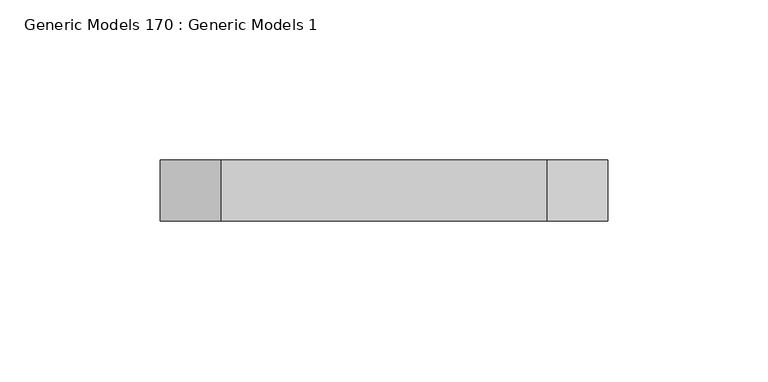
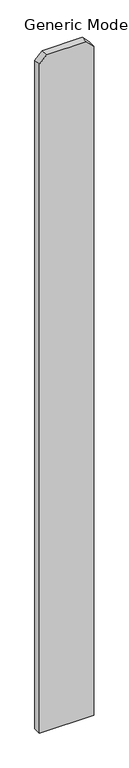
"""IFC4 building model written with IfcOpenShell, lengths in millimetres: proxy geometry, Generic Models 170 : Generic Models 1."""

from ifc_helpers import new_model, si_unit, frame, origin, place, context, project, spatial, polyline, outline, extrude, source, transform, mapped, element, save


def generic_models_170_generic_models_1_cb0b62f2(model_context):
    return source(origin(), model_context, "Body", "SweptSolid", [
        extrude(outline(polyline([(76.2, -248896.1875), (1885.95, -248896.1875), (1905.0, -248915.2375), (1905.0, -249016.8375), (1885.95, -249035.8875), (76.2, -249035.8875), (76.2, -248896.1875)])), frame((0.0, 547.6875, 0.0), z_axis=(0.0, 1.0, 0.0), x_axis=(0.0, 0.0, 1.0)), (0.0, 0.0, 1.0), 19.05),
    ])


if __name__ == "__main__":
    model = new_model("IFC4")
    model_context = context("Model", 3, world=origin())
    ifc_project = project(units=[si_unit("LENGTHUNIT", "METRE", prefix="MILLI")], contexts=[model_context])
    site = spatial("IfcSite", under=ifc_project)
    building = spatial("IfcBuilding", under=site)
    placement = place(None, origin())
    generic_models_170_generic_models_1_shape = generic_models_170_generic_models_1_cb0b62f2(model_context)
    element("IfcBuildingElementProxy", 1, Name="Generic Models 170 : Generic Models 1", ObjectType="Generic Models 170 : Generic Models 1", at=placement, inside=building, context=model_context, shape_type="MappedRepresentation", body=[
        mapped(generic_models_170_generic_models_1_shape, transform((0.0, 0.0, 0.0), x_axis=(1.0, 0.0, 0.0), y_axis=(0.0, 1.0, 0.0), z_axis=(0.0, 0.0, 1.0))),
    ])
    save(model, "model.ifc")

# Revit data of these elements
# Element 1 (IfcBuildingElementProxy, "Generic Models 170 : Generic Models 1")
#   Materials on its faces: "VERTICAL 1X6 CEDAR PLANKS W/ CLEAR WOOD SEALER"
# Materials
#   "VERTICAL 1X6 CEDAR PLANKS W/ CLEAR WOOD SEALER": class "Wood", colour RGB 234 198 147, transparency 0, Description = "Pinus Echinata", Cost = 0
